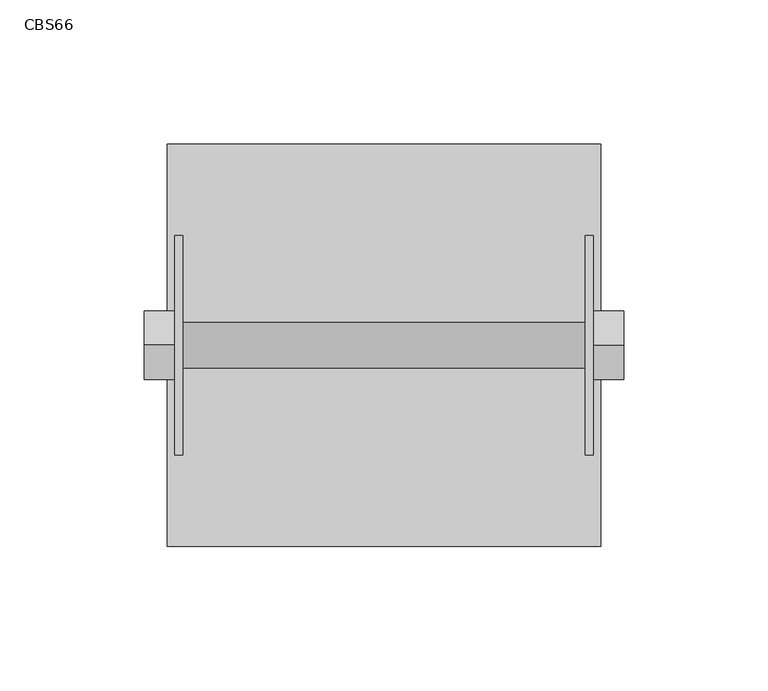
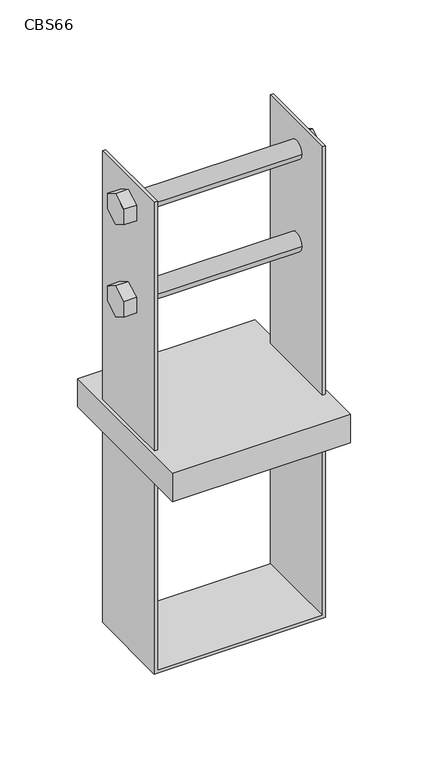
"""IFC4 building model written with IfcOpenShell, lengths in millimetres: fastener geometry, 060523 - W_P_C - Fastenings - Column Base - Simpson - CBS : CBS66."""

from ifc_helpers import new_model, si_unit, point, frame, frame_2d, origin, origin_with_axes, place, context, project, spatial, polyline, circle_curve, trimmed, segment, composite_curve, outline, extrude, source, transform, mapped, element, save


def cbs66_6cc2ebc6(model_context):
    return source(origin(), model_context, "Body", "SweptSolid", [
        extrude(outline(polyline([(11.90625, 132.8259234), (0.0, 125.9518467), (-11.90625, 132.8259234), (-11.90625, 146.5740766), (0.0, 153.4481533), (11.90625, 146.5740766), (11.90625, 132.8259234)])), frame((72.5289063, 0.0, 0.0), z_axis=(1.0, 0.0, 0.0), x_axis=(0.0, 1.0, 0.0)), (0.0, 0.0, 1.0), 10.715625),
        extrude(outline(polyline([(11.90625, 146.5740766), (11.90625, 132.8259234), (0.0, 125.9518467), (-11.90625, 132.8259234), (-11.90625, 146.5740766), (0.0, 153.4481533), (11.90625, 146.5740766)])), frame((-83.2445313, 0.0, 0.0), z_axis=(1.0, 0.0, 0.0), x_axis=(0.0, 1.0, 0.0)), (0.0, 0.0, 1.0), 10.715625),
        extrude(outline(composite_curve([segment(trimmed(circle_curve(frame_2d((0.0, 139.7)), 7.9375), [point((7.9375, 139.7))], [point((-7.9375, 139.7))], False, "CARTESIAN"), True, "CONTINUOUS"), segment(trimmed(circle_curve(frame_2d((0.0, 139.7)), 7.9375), [point((-7.9375, 139.7))], [point((7.9375, 139.7))], False, "CARTESIAN"), True, "CONTINUOUS")], self_intersect=False)), frame((-72.5289062, 0.0, 0.0), z_axis=(1.0, 0.0, 0.0), x_axis=(0.0, 1.0, 0.0)), (0.0, 0.0, 1.0), 152.4),
        extrude(outline(polyline([(11.90625, 215.3759234), (0.0, 208.5018467), (-11.90625, 215.3759234), (-11.90625, 229.1240766), (0.0, 235.9981533), (11.90625, 229.1240766), (11.90625, 215.3759234)])), frame((72.5289063, 0.0, 0.0), z_axis=(1.0, 0.0, 0.0), x_axis=(0.0, 1.0, 0.0)), (0.0, 0.0, 1.0), 10.715625),
        extrude(outline(polyline([(11.90625, 229.1240766), (11.90625, 215.3759234), (0.0, 208.5018467), (-11.90625, 215.3759234), (-11.90625, 229.1240766), (0.0, 235.9981533), (11.90625, 229.1240766)])), frame((-83.2445313, 0.0, 0.0), z_axis=(1.0, 0.0, 0.0), x_axis=(0.0, 1.0, 0.0)), (0.0, 0.0, 1.0), 10.715625),
        extrude(outline(composite_curve([segment(trimmed(circle_curve(frame_2d((0.0, 222.25)), 7.9375), [point((7.9375, 222.25))], [point((-7.9375, 222.25))], False, "CARTESIAN"), True, "CONTINUOUS"), segment(trimmed(circle_curve(frame_2d((0.0, 222.25)), 7.9375), [point((-7.9375, 222.25))], [point((7.9375, 222.25))], False, "CARTESIAN"), True, "CONTINUOUS")], self_intersect=False)), frame((-72.5289062, 0.0, 0.0), z_axis=(1.0, 0.0, 0.0), x_axis=(0.0, 1.0, 0.0)), (0.0, 0.0, 1.0), 152.4),
        extrude(outline(polyline([(-174.625, 72.5289063), (247.65, 72.5289063), (247.65, 69.85), (-171.9460938, 69.85), (-171.9460938, -69.85), (247.65, -69.85), (247.65, -72.5289062), (-174.625, -72.5289062), (-174.625, 72.5289063)])), frame((0.0, -38.1, 0.0), z_axis=(0.0, 1.0, 0.0), x_axis=(0.0, 0.0, 1.0)), (0.0, 0.0, 1.0), 76.2),
        extrude(outline(polyline([(75.2078125, 69.85), (75.2078125, -69.85), (-75.2078125, -69.85), (-75.2078125, 69.85), (75.2078125, 69.85)])), origin_with_axes(), (0.0, 0.0, 1.0), 25.4),
    ])


if __name__ == "__main__":
    model = new_model("IFC4")
    model_context = context("Model", 3, world=origin())
    ifc_project = project(units=[si_unit("LENGTHUNIT", "METRE", prefix="MILLI")], contexts=[model_context])
    site = spatial("IfcSite", under=ifc_project)
    building = spatial("IfcBuilding", under=site)
    placement = place(None, origin())
    cbs66_shape = cbs66_6cc2ebc6(model_context)
    element("IfcFastener", 1, ObjectType="060523 - W_P_C - Fastenings - Column Base - Simpson - CBS : CBS66", at=placement, inside=building, context=model_context, shape_type="MappedRepresentation", body=[
        mapped(cbs66_shape, transform((0.0, 0.0, 0.0), x_axis=(1.0, 0.0, 0.0), y_axis=(0.0, 1.0, 0.0), z_axis=(0.0, 0.0, 1.0))),
    ])
    save(model, "model.ifc")

# Revit data of these elements
# Type "060523 - W_P_C - Fastenings - Column Base - Simpson - CBS : CBS66"
#   W2 = 0' - 5 1/2"
#   W1 = 0' - 5 1/2"
#   H = 0' - 8 3/4"
#   Gauge = 0' - 0 27/256"
#   Flange Width = 0' - 3"
#   D = 0' - 6 7/8"
#   Material = SIMPSON CBS66 COLUMN BASE (RAW STEEL - SPECIAL ORDER)
# Element 1 (IfcFastener, "060523 - W_P_C - Fastenings - Column Base - Simpson - CBS : CBS66")
#   Materials on its faces: "STRUCTURAL BOLTS (PAINT TO MATCH STEEL FINISH)", "SIMPSON CBS66 COLUMN BASE (RAW STEEL - SPECIAL ORDER)"
# Materials
#   "SIMPSON CBS66 COLUMN BASE (RAW STEEL - SPECIAL ORDER)": class "Generic", colour RGB 212 212 212, transparency 0, Cost = 0
#   "STRUCTURAL BOLTS (PAINT TO MATCH STEEL FINISH)": class "Generic", colour RGB 120 120 120, transparency 0, Cost = 0
